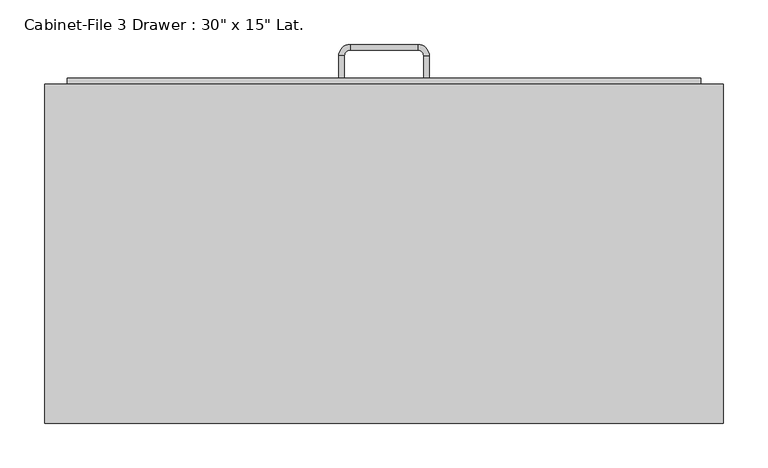
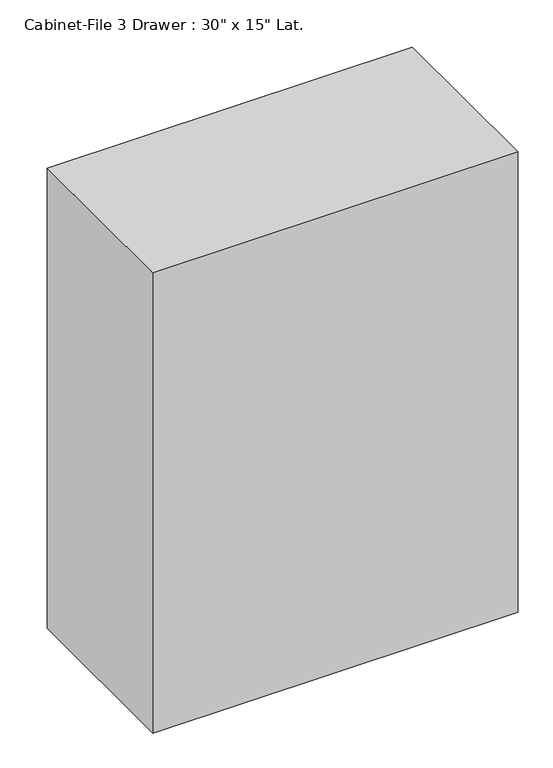
"""IFC4 building model written with IfcOpenShell, lengths in millimetres: furniture geometry."""

from ifc_helpers import new_model, si_unit, frame, origin, origin_with_axes, place, context, project, spatial, polyline, circle_curve, outline, extrude, source, transform, mapped, element, save
from ifc_brep_helpers import plane_surface, cylinder_surface, revolved_surface, advanced_brep


def furniture_5292397e(model_context):
    return source(origin(), model_context, "Body", "SolidModel", [
        extrude(outline(polyline([(253.103553, -48.3656999), (-508.896447, -48.3656999), (-508.896447, 332.6343001), (253.103553, 332.6343001), (253.103553, -48.3656999)])), origin_with_axes(), (0.0, 0.0, 1.0), 1016.0),
        extrude(outline(polyline([(227.703553, 338.9843001), (227.703553, 332.6343001), (-483.496447, 332.6343001), (-483.496447, 338.9843001), (227.703553, 338.9843001)])), frame((0.0, 0.0, 736.6), z_axis=(0.0, 0.0, 1.0), x_axis=(1.0, 0.0, 0.0)), (0.0, 0.0, 1.0), 254.0),
        extrude(outline(polyline([(227.703553, 338.9843001), (227.703553, 332.6343001), (-483.496447, 332.6343001), (-483.496447, 338.9843001), (227.703553, 338.9843001)])), frame((0.0, 0.0, 431.8), z_axis=(0.0, 0.0, 1.0), x_axis=(1.0, 0.0, 0.0)), (0.0, 0.0, 1.0), 279.4),
        extrude(outline(polyline([(227.703553, 338.9843001), (227.703553, 332.6343001), (-483.496447, 332.6343001), (-483.496447, 338.9843001), (227.703553, 338.9843001)])), frame((0.0, 0.0, 127.0), z_axis=(0.0, 0.0, 1.0), x_axis=(1.0, 0.0, 0.0)), (0.0, 0.0, 1.0), 279.4),
        advanced_brep(
        [(-172.346447, 338.9843001, 203.2), (-172.346447, 338.9843001, 215.9), (-178.696447, 338.9843001, 215.9), (-178.696447, 338.9843001, 203.2), (-178.696447, 364.3843001, 203.2), (-172.346447, 364.3843001, 203.2), (-178.696447, 364.3843001, 215.9), (-172.346447, 364.3843001, 215.9), (-165.996447, 377.0843001, 203.2), (-165.996447, 370.7343001, 203.2), (-165.996447, 377.0843001, 215.9), (-165.996447, 370.7343001, 215.9), (-89.796447, 377.0843001, 203.2), (-89.796447, 370.7343001, 203.2), (-89.796447, 377.0843001, 215.9), (-89.796447, 370.7343001, 215.9), (-77.096447, 364.3843001, 203.2), (-83.446447, 364.3843001, 203.2), (-77.096447, 364.3843001, 215.9), (-83.446447, 364.3843001, 215.9), (-83.446447, 338.9843001, 203.2), (-77.096447, 338.9843001, 203.2), (-77.096447, 338.9843001, 215.9), (-83.446447, 338.9843001, 215.9)],
        [
            (0, 1),
            (1, 2),
            (2, 3),
            (3, 0),
            (3, 4),
            (4, 5),
            (5, 0),
            (2, 6),
            (6, 4),
            (1, 7),
            (7, 6),
            (5, 7),
            (8, 9),
            (9, 5, circle_curve(frame((-165.996447, 364.3843001, 203.2), z_axis=(0.0, 0.0, 1.0), x_axis=(-1.0, 0.0, 0.0)), 6.35)),
            (4, 8, circle_curve(frame((-165.996447, 364.3843001, 203.2), z_axis=(0.0, 0.0, -1.0), x_axis=(-1.0, 0.0, 0.0)), 12.7)),
            (10, 8),
            (6, 10, circle_curve(frame((-165.996447, 364.3843001, 215.9), z_axis=(0.0, 0.0, -1.0), x_axis=(-1.0, 0.0, 0.0)), 12.7)),
            (11, 10),
            (7, 11, circle_curve(frame((-165.996447, 364.3843001, 215.9), z_axis=(0.0, 0.0, -1.0), x_axis=(-1.0, 0.0, 0.0)), 6.35)),
            (9, 11),
            (8, 12),
            (12, 13),
            (13, 9),
            (10, 14),
            (14, 12),
            (11, 15),
            (15, 14),
            (13, 15),
            (16, 17),
            (17, 13, circle_curve(frame((-89.796447, 364.3843001, 203.2), z_axis=(0.0, 0.0, 1.0), x_axis=(0.0, 1.0, 0.0)), 6.35)),
            (12, 16, circle_curve(frame((-89.796447, 364.3843001, 203.2), z_axis=(0.0, 0.0, -1.0), x_axis=(0.0, 1.0, 0.0)), 12.7)),
            (18, 16),
            (14, 18, circle_curve(frame((-89.796447, 364.3843001, 215.9), z_axis=(0.0, 0.0, -1.0), x_axis=(0.0, 1.0, 0.0)), 12.7)),
            (19, 18),
            (15, 19, circle_curve(frame((-89.796447, 364.3843001, 215.9), z_axis=(0.0, 0.0, -1.0), x_axis=(0.0, 1.0, 0.0)), 6.35)),
            (17, 19),
            (20, 21),
            (21, 22),
            (22, 23),
            (23, 20),
            (16, 21),
            (20, 17),
            (18, 22),
            (19, 23),
        ],
        [
            plane_surface(frame((-978.8216451, 338.9843001, 0.0), z_axis=(0.0, -1.0, 0.0), x_axis=(0.0, 0.0, -1.0))),
            plane_surface(frame((-172.346447, 338.9843001, 203.2), z_axis=(0.0, 0.0, -1.0), x_axis=(0.0, 1.0, 0.0))),
            plane_surface(frame((-178.696447, 338.9843001, 203.2), z_axis=(-1.0, 0.0, 0.0), x_axis=(0.0, 1.0, 0.0))),
            plane_surface(frame((-178.696447, 338.9843001, 215.9), z_axis=(0.0, 0.0, 1.0), x_axis=(0.0, 1.0, 0.0))),
            plane_surface(frame((-172.346447, 338.9843001, 215.9), z_axis=(1.0, 0.0, 0.0), x_axis=(0.0, 1.0, 0.0))),
            plane_surface(frame((-165.996447, 364.3843001, 203.2), z_axis=(0.0, 0.0, -1.0), x_axis=(-1.0, 0.0, 0.0))),
            cylinder_surface(frame((-165.996447, 364.3843001, 0.0), z_axis=(0.0, 0.0, 1.0), x_axis=(-1.0, 0.0, 0.0)), 12.7),
            plane_surface(frame((-165.996447, 364.3843001, 215.9), z_axis=(0.0, 0.0, 1.0), x_axis=(-1.0, 0.0, 0.0))),
            revolved_surface(polyline([(-172.34644699999998, 364.3843001, 215.9), (-172.34644699999998, 364.3843001, 203.2)]), (-165.996447, 364.3843001, 0.0), (0.0, 0.0, 1.0)),
            plane_surface(frame((-165.996447, 370.7343001, 203.2), z_axis=(0.0, 0.0, -1.0), x_axis=(1.0, 0.0, 0.0))),
            plane_surface(frame((-165.996447, 377.0843001, 203.2), z_axis=(0.0, 1.0, 0.0), x_axis=(1.0, 0.0, 0.0))),
            plane_surface(frame((-165.996447, 377.0843001, 215.9), z_axis=(0.0, 0.0, 1.0), x_axis=(1.0, 0.0, 0.0))),
            plane_surface(frame((-165.996447, 370.7343001, 215.9), z_axis=(0.0, -1.0, 0.0), x_axis=(1.0, 0.0, 0.0))),
            plane_surface(frame((-89.796447, 364.3843001, 203.2), z_axis=(0.0, 0.0, -1.0), x_axis=(0.0, 1.0, 0.0))),
            cylinder_surface(frame((-89.796447, 364.3843001, 0.0), z_axis=(0.0, 0.0, 1.0), x_axis=(0.0, 1.0, 0.0)), 12.7),
            plane_surface(frame((-89.796447, 364.3843001, 215.9), z_axis=(0.0, 0.0, 1.0), x_axis=(0.0, 1.0, 0.0))),
            revolved_surface(polyline([(-89.796447, 370.73430010000004, 215.9), (-89.796447, 370.73430010000004, 203.2)]), (-89.796447, 364.3843001, 0.0), (0.0, 0.0, 1.0)),
            plane_surface(frame((-877.2216451, 338.9843001, 0.0), z_axis=(0.0, -1.0, 0.0), x_axis=(0.0, 0.0, 1.0))),
            plane_surface(frame((-83.446447, 364.3843001, 203.2), z_axis=(0.0, 0.0, -1.0), x_axis=(0.0, -1.0, 0.0))),
            plane_surface(frame((-77.096447, 364.3843001, 203.2), z_axis=(1.0, 0.0, 0.0), x_axis=(0.0, -1.0, 0.0))),
            plane_surface(frame((-77.096447, 364.3843001, 215.9), z_axis=(0.0, 0.0, 1.0), x_axis=(0.0, -1.0, 0.0))),
            plane_surface(frame((-83.446447, 364.3843001, 215.9), z_axis=(-1.0, 0.0, 0.0), x_axis=(0.0, -1.0, 0.0))),
        ],
        [
            (0, [[1, 2, 3, 4]]),
            (1, [[5, 6, 7, -4]]),
            (2, [[8, 9, -5, -3]]),
            (3, [[10, 11, -8, -2]]),
            (4, [[-7, 12, -10, -1]]),
            (5, [[13, 14, -6, 15]]),
            (6, [[16, -15, -9, 17]]),
            (7, [[18, -17, -11, 19]]),
            (8, [[20, -19, -12, -14]]),
            (9, [[21, 22, 23, -13]]),
            (10, [[24, 25, -21, -16]]),
            (11, [[26, 27, -24, -18]]),
            (12, [[-23, 28, -26, -20]]),
            (13, [[29, 30, -22, 31]]),
            (14, [[32, -31, -25, 33]]),
            (15, [[34, -33, -27, 35]]),
            (16, [[36, -35, -28, -30]]),
            (17, [[37, 38, 39, 40]]),
            (18, [[41, -37, 42, -29]]),
            (19, [[43, -38, -41, -32]]),
            (20, [[44, -39, -43, -34]]),
            (21, [[-42, -40, -44, -36]]),
        ],
    ),
        advanced_brep(
        [(-172.346447, 338.9843001, 482.6), (-172.346447, 338.9843001, 495.3), (-178.696447, 338.9843001, 495.3), (-178.696447, 338.9843001, 482.6), (-178.696447, 364.3843001, 482.6), (-172.346447, 364.3843001, 482.6), (-178.696447, 364.3843001, 495.3), (-172.346447, 364.3843001, 495.3), (-165.996447, 377.0843001, 482.6), (-165.996447, 370.7343001, 482.6), (-165.996447, 377.0843001, 495.3), (-165.996447, 370.7343001, 495.3), (-89.796447, 377.0843001, 482.6), (-89.796447, 370.7343001, 482.6), (-89.796447, 377.0843001, 495.3), (-89.796447, 370.7343001, 495.3), (-77.096447, 364.3843001, 482.6), (-83.446447, 364.3843001, 482.6), (-77.096447, 364.3843001, 495.3), (-83.446447, 364.3843001, 495.3), (-83.446447, 338.9843001, 482.6), (-77.096447, 338.9843001, 482.6), (-77.096447, 338.9843001, 495.3), (-83.446447, 338.9843001, 495.3)],
        [
            (0, 1),
            (1, 2),
            (2, 3),
            (3, 0),
            (3, 4),
            (4, 5),
            (5, 0),
            (2, 6),
            (6, 4),
            (1, 7),
            (7, 6),
            (5, 7),
            (8, 9),
            (9, 5, circle_curve(frame((-165.996447, 364.3843001, 482.6), z_axis=(0.0, 0.0, 1.0), x_axis=(-1.0, 0.0, 0.0)), 6.35)),
            (4, 8, circle_curve(frame((-165.996447, 364.3843001, 482.6), z_axis=(0.0, 0.0, -1.0), x_axis=(-1.0, 0.0, 0.0)), 12.7)),
            (10, 8),
            (6, 10, circle_curve(frame((-165.996447, 364.3843001, 495.3), z_axis=(0.0, 0.0, -1.0), x_axis=(-1.0, 0.0, 0.0)), 12.7)),
            (11, 10),
            (7, 11, circle_curve(frame((-165.996447, 364.3843001, 495.3), z_axis=(0.0, 0.0, -1.0), x_axis=(-1.0, 0.0, 0.0)), 6.35)),
            (9, 11),
            (8, 12),
            (12, 13),
            (13, 9),
            (10, 14),
            (14, 12),
            (11, 15),
            (15, 14),
            (13, 15),
            (16, 17),
            (17, 13, circle_curve(frame((-89.796447, 364.3843001, 482.6), z_axis=(0.0, 0.0, 1.0), x_axis=(0.0, 1.0, 0.0)), 6.35)),
            (12, 16, circle_curve(frame((-89.796447, 364.3843001, 482.6), z_axis=(0.0, 0.0, -1.0), x_axis=(0.0, 1.0, 0.0)), 12.7)),
            (18, 16),
            (14, 18, circle_curve(frame((-89.796447, 364.3843001, 495.3), z_axis=(0.0, 0.0, -1.0), x_axis=(0.0, 1.0, 0.0)), 12.7)),
            (19, 18),
            (15, 19, circle_curve(frame((-89.796447, 364.3843001, 495.3), z_axis=(0.0, 0.0, -1.0), x_axis=(0.0, 1.0, 0.0)), 6.35)),
            (17, 19),
            (20, 21),
            (21, 22),
            (22, 23),
            (23, 20),
            (16, 21),
            (20, 17),
            (18, 22),
            (19, 23),
        ],
        [
            plane_surface(frame((-978.8216451, 338.9843001, 0.0), z_axis=(0.0, -1.0, 0.0), x_axis=(0.0, 0.0, -1.0))),
            plane_surface(frame((-172.346447, 338.9843001, 482.6), z_axis=(0.0, 0.0, -1.0), x_axis=(0.0, 1.0, 0.0))),
            plane_surface(frame((-178.696447, 338.9843001, 482.6), z_axis=(-1.0, 0.0, 0.0), x_axis=(0.0, 1.0, 0.0))),
            plane_surface(frame((-178.696447, 338.9843001, 495.3), z_axis=(0.0, 0.0, 1.0), x_axis=(0.0, 1.0, 0.0))),
            plane_surface(frame((-172.346447, 338.9843001, 495.3), z_axis=(1.0, 0.0, 0.0), x_axis=(0.0, 1.0, 0.0))),
            plane_surface(frame((-165.996447, 364.3843001, 482.6), z_axis=(0.0, 0.0, -1.0), x_axis=(-1.0, 0.0, 0.0))),
            cylinder_surface(frame((-165.996447, 364.3843001, 0.0), z_axis=(0.0, 0.0, 1.0), x_axis=(-1.0, 0.0, 0.0)), 12.7),
            plane_surface(frame((-165.996447, 364.3843001, 495.3), z_axis=(0.0, 0.0, 1.0), x_axis=(-1.0, 0.0, 0.0))),
            revolved_surface(polyline([(-172.34644699999998, 364.3843001, 495.3), (-172.34644699999998, 364.3843001, 482.6)]), (-165.996447, 364.3843001, 0.0), (0.0, 0.0, 1.0)),
            plane_surface(frame((-165.996447, 370.7343001, 482.6), z_axis=(0.0, 0.0, -1.0), x_axis=(1.0, 0.0, 0.0))),
            plane_surface(frame((-165.996447, 377.0843001, 482.6), z_axis=(0.0, 1.0, 0.0), x_axis=(1.0, 0.0, 0.0))),
            plane_surface(frame((-165.996447, 377.0843001, 495.3), z_axis=(0.0, 0.0, 1.0), x_axis=(1.0, 0.0, 0.0))),
            plane_surface(frame((-165.996447, 370.7343001, 495.3), z_axis=(0.0, -1.0, 0.0), x_axis=(1.0, 0.0, 0.0))),
            plane_surface(frame((-89.796447, 364.3843001, 482.6), z_axis=(0.0, 0.0, -1.0), x_axis=(0.0, 1.0, 0.0))),
            cylinder_surface(frame((-89.796447, 364.3843001, 0.0), z_axis=(0.0, 0.0, 1.0), x_axis=(0.0, 1.0, 0.0)), 12.7),
            plane_surface(frame((-89.796447, 364.3843001, 495.3), z_axis=(0.0, 0.0, 1.0), x_axis=(0.0, 1.0, 0.0))),
            revolved_surface(polyline([(-89.796447, 370.73430010000004, 495.3), (-89.796447, 370.73430010000004, 482.6)]), (-89.796447, 364.3843001, 0.0), (0.0, 0.0, 1.0)),
            plane_surface(frame((-877.2216451, 338.9843001, 0.0), z_axis=(0.0, -1.0, 0.0), x_axis=(0.0, 0.0, 1.0))),
            plane_surface(frame((-83.446447, 364.3843001, 482.6), z_axis=(0.0, 0.0, -1.0), x_axis=(0.0, -1.0, 0.0))),
            plane_surface(frame((-77.096447, 364.3843001, 482.6), z_axis=(1.0, 0.0, 0.0), x_axis=(0.0, -1.0, 0.0))),
            plane_surface(frame((-77.096447, 364.3843001, 495.3), z_axis=(0.0, 0.0, 1.0), x_axis=(0.0, -1.0, 0.0))),
            plane_surface(frame((-83.446447, 364.3843001, 495.3), z_axis=(-1.0, 0.0, 0.0), x_axis=(0.0, -1.0, 0.0))),
        ],
        [
            (0, [[1, 2, 3, 4]]),
            (1, [[5, 6, 7, -4]]),
            (2, [[8, 9, -5, -3]]),
            (3, [[10, 11, -8, -2]]),
            (4, [[-7, 12, -10, -1]]),
            (5, [[13, 14, -6, 15]]),
            (6, [[16, -15, -9, 17]]),
            (7, [[18, -17, -11, 19]]),
            (8, [[20, -19, -12, -14]]),
            (9, [[21, 22, 23, -13]]),
            (10, [[24, 25, -21, -16]]),
            (11, [[26, 27, -24, -18]]),
            (12, [[-23, 28, -26, -20]]),
            (13, [[29, 30, -22, 31]]),
            (14, [[32, -31, -25, 33]]),
            (15, [[34, -33, -27, 35]]),
            (16, [[36, -35, -28, -30]]),
            (17, [[37, 38, 39, 40]]),
            (18, [[41, -37, 42, -29]]),
            (19, [[43, -38, -41, -32]]),
            (20, [[44, -39, -43, -34]]),
            (21, [[-42, -40, -44, -36]]),
        ],
    ),
        advanced_brep(
        [(-172.346447, 338.9843001, 787.4), (-172.346447, 338.9843001, 800.1), (-178.696447, 338.9843001, 800.1), (-178.696447, 338.9843001, 787.4), (-178.696447, 364.3843001, 787.4), (-172.346447, 364.3843001, 787.4), (-178.696447, 364.3843001, 800.1), (-172.346447, 364.3843001, 800.1), (-165.996447, 377.0843001, 787.4), (-165.996447, 370.7343001, 787.4), (-165.996447, 377.0843001, 800.1), (-165.996447, 370.7343001, 800.1), (-89.796447, 377.0843001, 787.4), (-89.796447, 370.7343001, 787.4), (-89.796447, 377.0843001, 800.1), (-89.796447, 370.7343001, 800.1), (-77.096447, 364.3843001, 787.4), (-83.446447, 364.3843001, 787.4), (-77.096447, 364.3843001, 800.1), (-83.446447, 364.3843001, 800.1), (-83.446447, 338.9843001, 787.4), (-77.096447, 338.9843001, 787.4), (-77.096447, 338.9843001, 800.1), (-83.446447, 338.9843001, 800.1)],
        [
            (0, 1),
            (1, 2),
            (2, 3),
            (3, 0),
            (3, 4),
            (4, 5),
            (5, 0),
            (2, 6),
            (6, 4),
            (1, 7),
            (7, 6),
            (5, 7),
            (8, 9),
            (9, 5, circle_curve(frame((-165.996447, 364.3843001, 787.4), z_axis=(0.0, 0.0, 1.0), x_axis=(-1.0, 0.0, 0.0)), 6.35)),
            (4, 8, circle_curve(frame((-165.996447, 364.3843001, 787.4), z_axis=(0.0, 0.0, -1.0), x_axis=(-1.0, 0.0, 0.0)), 12.7)),
            (10, 8),
            (6, 10, circle_curve(frame((-165.996447, 364.3843001, 800.1), z_axis=(0.0, 0.0, -1.0), x_axis=(-1.0, 0.0, 0.0)), 12.7)),
            (11, 10),
            (7, 11, circle_curve(frame((-165.996447, 364.3843001, 800.1), z_axis=(0.0, 0.0, -1.0), x_axis=(-1.0, 0.0, 0.0)), 6.35)),
            (9, 11),
            (8, 12),
            (12, 13),
            (13, 9),
            (10, 14),
            (14, 12),
            (11, 15),
            (15, 14),
            (13, 15),
            (16, 17),
            (17, 13, circle_curve(frame((-89.796447, 364.3843001, 787.4), z_axis=(0.0, 0.0, 1.0), x_axis=(0.0, 1.0, 0.0)), 6.35)),
            (12, 16, circle_curve(frame((-89.796447, 364.3843001, 787.4), z_axis=(0.0, 0.0, -1.0), x_axis=(0.0, 1.0, 0.0)), 12.7)),
            (18, 16),
            (14, 18, circle_curve(frame((-89.796447, 364.3843001, 800.1), z_axis=(0.0, 0.0, -1.0), x_axis=(0.0, 1.0, 0.0)), 12.7)),
            (19, 18),
            (15, 19, circle_curve(frame((-89.796447, 364.3843001, 800.1), z_axis=(0.0, 0.0, -1.0), x_axis=(0.0, 1.0, 0.0)), 6.35)),
            (17, 19),
            (20, 21),
            (21, 22),
            (22, 23),
            (23, 20),
            (16, 21),
            (20, 17),
            (18, 22),
            (19, 23),
        ],
        [
            plane_surface(frame((-978.8216451, 338.9843001, 0.0), z_axis=(0.0, -1.0, 0.0), x_axis=(0.0, 0.0, -1.0))),
            plane_surface(frame((-172.346447, 338.9843001, 787.4), z_axis=(0.0, 0.0, -1.0), x_axis=(0.0, 1.0, 0.0))),
            plane_surface(frame((-178.696447, 338.9843001, 787.4), z_axis=(-1.0, 0.0, 0.0), x_axis=(0.0, 1.0, 0.0))),
            plane_surface(frame((-178.696447, 338.9843001, 800.1), z_axis=(0.0, 0.0, 1.0), x_axis=(0.0, 1.0, 0.0))),
            plane_surface(frame((-172.346447, 338.9843001, 800.1), z_axis=(1.0, 0.0, 0.0), x_axis=(0.0, 1.0, 0.0))),
            plane_surface(frame((-165.996447, 364.3843001, 787.4), z_axis=(0.0, 0.0, -1.0), x_axis=(-1.0, 0.0, 0.0))),
            cylinder_surface(frame((-165.996447, 364.3843001, 0.0), z_axis=(0.0, 0.0, 1.0), x_axis=(-1.0, 0.0, 0.0)), 12.7),
            plane_surface(frame((-165.996447, 364.3843001, 800.1), z_axis=(0.0, 0.0, 1.0), x_axis=(-1.0, 0.0, 0.0))),
            revolved_surface(polyline([(-172.34644699999998, 364.3843001, 800.1), (-172.34644699999998, 364.3843001, 787.4)]), (-165.996447, 364.3843001, 0.0), (0.0, 0.0, 1.0)),
            plane_surface(frame((-165.996447, 370.7343001, 787.4), z_axis=(0.0, 0.0, -1.0), x_axis=(1.0, 0.0, 0.0))),
            plane_surface(frame((-165.996447, 377.0843001, 787.4), z_axis=(0.0, 1.0, 0.0), x_axis=(1.0, 0.0, 0.0))),
            plane_surface(frame((-165.996447, 377.0843001, 800.1), z_axis=(0.0, 0.0, 1.0), x_axis=(1.0, 0.0, 0.0))),
            plane_surface(frame((-165.996447, 370.7343001, 800.1), z_axis=(0.0, -1.0, 0.0), x_axis=(1.0, 0.0, 0.0))),
            plane_surface(frame((-89.796447, 364.3843001, 787.4), z_axis=(0.0, 0.0, -1.0), x_axis=(0.0, 1.0, 0.0))),
            cylinder_surface(frame((-89.796447, 364.3843001, 0.0), z_axis=(0.0, 0.0, 1.0), x_axis=(0.0, 1.0, 0.0)), 12.7),
            plane_surface(frame((-89.796447, 364.3843001, 800.1), z_axis=(0.0, 0.0, 1.0), x_axis=(0.0, 1.0, 0.0))),
            revolved_surface(polyline([(-89.796447, 370.73430010000004, 800.1), (-89.796447, 370.73430010000004, 787.4)]), (-89.796447, 364.3843001, 0.0), (0.0, 0.0, 1.0)),
            plane_surface(frame((-877.2216451, 338.9843001, 0.0), z_axis=(0.0, -1.0, 0.0), x_axis=(0.0, 0.0, 1.0))),
            plane_surface(frame((-83.446447, 364.3843001, 787.4), z_axis=(0.0, 0.0, -1.0), x_axis=(0.0, -1.0, 0.0))),
            plane_surface(frame((-77.096447, 364.3843001, 787.4), z_axis=(1.0, 0.0, 0.0), x_axis=(0.0, -1.0, 0.0))),
            plane_surface(frame((-77.096447, 364.3843001, 800.1), z_axis=(0.0, 0.0, 1.0), x_axis=(0.0, -1.0, 0.0))),
            plane_surface(frame((-83.446447, 364.3843001, 800.1), z_axis=(-1.0, 0.0, 0.0), x_axis=(0.0, -1.0, 0.0))),
        ],
        [
            (0, [[1, 2, 3, 4]]),
            (1, [[5, 6, 7, -4]]),
            (2, [[8, 9, -5, -3]]),
            (3, [[10, 11, -8, -2]]),
            (4, [[-7, 12, -10, -1]]),
            (5, [[13, 14, -6, 15]]),
            (6, [[16, -15, -9, 17]]),
            (7, [[18, -17, -11, 19]]),
            (8, [[20, -19, -12, -14]]),
            (9, [[21, 22, 23, -13]]),
            (10, [[24, 25, -21, -16]]),
            (11, [[26, 27, -24, -18]]),
            (12, [[-23, 28, -26, -20]]),
            (13, [[29, 30, -22, 31]]),
            (14, [[32, -31, -25, 33]]),
            (15, [[34, -33, -27, 35]]),
            (16, [[36, -35, -28, -30]]),
            (17, [[37, 38, 39, 40]]),
            (18, [[41, -37, 42, -29]]),
            (19, [[43, -38, -41, -32]]),
            (20, [[44, -39, -43, -34]]),
            (21, [[-42, -40, -44, -36]]),
        ],
    ),
    ])


if __name__ == "__main__":
    model = new_model("IFC4")
    model_context = context("Model", 3, world=origin())
    ifc_project = project(units=[si_unit("LENGTHUNIT", "METRE", prefix="MILLI")], contexts=[model_context])
    site = spatial("IfcSite", under=ifc_project)
    building = spatial("IfcBuilding", under=site)
    placement = place(None, origin())
    furniture_shape = furniture_5292397e(model_context)
    element("IfcFurniture", 1, ObjectType="Cabinet-File 3 Drawer : 30\" x 15\" Lat.", at=placement, inside=building, context=model_context, shape_type="MappedRepresentation", body=[
        mapped(furniture_shape, transform((0.0, 0.0, 0.0), x_axis=(1.0, 0.0, 0.0), y_axis=(0.0, 1.0, 0.0), z_axis=(0.0, 0.0, 1.0))),
    ])
    save(model, "model.ifc")

# Revit data of these elements
# Type "Cabinet-File 3 Drawer : 30\" x 15\" Lat."
#   Assembly Code = "E2020200"
#   Depth = 1' - 3"
#   Height = 3' - 4"
#   Width = 2' - 6"
#   Cabinet Material = Steel, Paint Finish, Ivory, Glossy
#   Handle Material = Steel, Chrome Plated
#   Default Elevation = 0
# Element 1 (IfcFurniture, "Cabinet-File 3 Drawer : 30\" x 15\" Lat.")
#   Materials on its faces: "Steel, Chrome Plated", "Steel, Paint Finish, Ivory, Glossy"
# Materials
#   "Steel, Paint Finish, Ivory, Glossy": class "Metal", colour RGB 247 247 239, transparency 0, Description = "Steel, paint finish, ivory, glossy", Cost = 0
#   "Steel, Chrome Plated": class "Metal", colour RGB 17 17 17, transparency 0, Description = "Chromiuim plated steel", Cost = 0
